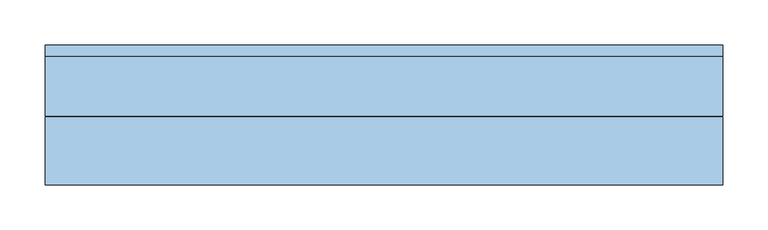
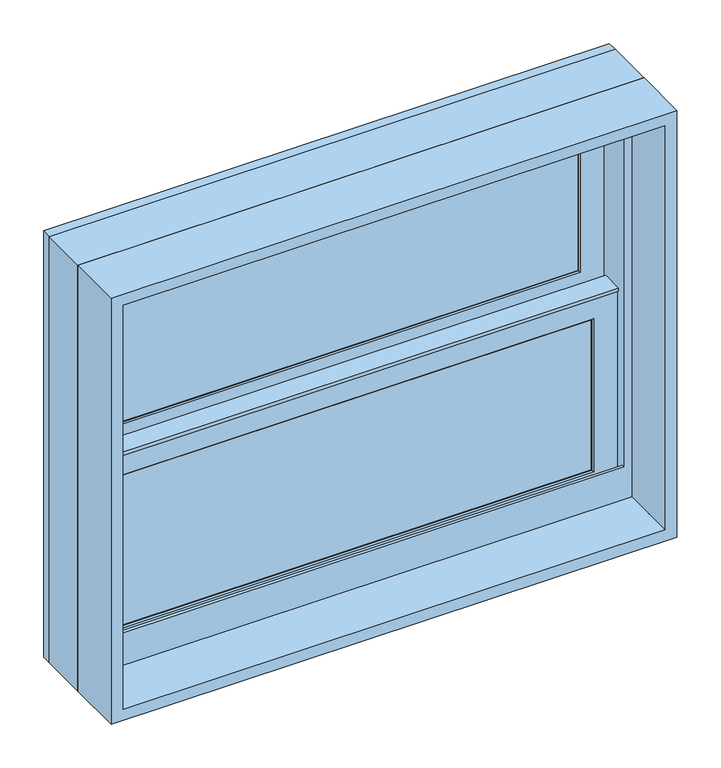
"""IFC4 building model written with IfcOpenShell, lengths in millimetres: window geometry, Window-Double_Hung-Marvin-Essential : ESDH2620."""

from ifc_helpers import new_model, si_unit, frame, origin, place, context, project, spatial, polyline, outline, extrude, faceted_brep, source, transform, mapped, element, save


def window_aca55058(model_context):
    return source(origin(), model_context, "Body", "SolidModel", [
        extrude(outline(polyline([(115.3583333, 20.6375), (115.3583333, 15.875), (96.3083333, 15.875), (96.3083333, 20.6375), (115.3583333, 20.6375)])), frame((0.0, 0.0, 1898.65), z_axis=(0.0, 0.0, 1.0), x_axis=(1.0, 0.0, 0.0)), (0.0, 0.0, 1.0), 222.25),
        extrude(outline(polyline([(-96.3083333, 20.6375), (-96.3083333, 15.875), (-115.3583333, 15.875), (-115.3583333, 20.6375), (-96.3083333, 20.6375)])), frame((0.0, 0.0, 1898.65), z_axis=(0.0, 0.0, 1.0), x_axis=(1.0, 0.0, 0.0)), (0.0, 0.0, 1.0), 222.25),
        extrude(outline(polyline([(317.5, 20.6375), (317.5, 15.875), (-317.5, 15.875), (-317.5, 20.6375), (317.5, 20.6375)])), frame((0.0, 0.0, 2000.25), z_axis=(0.0, 0.0, 1.0), x_axis=(1.0, 0.0, 0.0)), (0.0, 0.0, 1.0), 19.05),
        extrude(outline(polyline([(-115.3583333, 46.83125), (-115.3583333, 51.59375), (-96.3083333, 51.59375), (-96.3083333, 46.83125), (-115.3583333, 46.83125)])), frame((0.0, 0.0, 2159.0), z_axis=(0.0, 0.0, 1.0), x_axis=(1.0, 0.0, 0.0)), (0.0, 0.0, 1.0), 222.25),
        extrude(outline(polyline([(96.3083333, 46.83125), (96.3083333, 51.59375), (115.3583333, 51.59375), (115.3583333, 46.83125), (96.3083333, 46.83125)])), frame((0.0, 0.0, 2159.0), z_axis=(0.0, 0.0, 1.0), x_axis=(1.0, 0.0, 0.0)), (0.0, 0.0, 1.0), 222.25),
        extrude(outline(polyline([(-317.5, 46.83125), (-317.5, 51.59375), (317.5, 51.59375), (317.5, 46.83125), (-317.5, 46.83125)])), frame((0.0, 0.0, 2260.6), z_axis=(0.0, 0.0, 1.0), x_axis=(1.0, 0.0, 0.0)), (0.0, 0.0, 1.0), 19.05),
        extrude(outline(polyline([(115.3583333, 20.6375), (96.3083333, 20.6375), (96.3083333, 25.4), (115.3583333, 25.4), (115.3583333, 20.6375)])), frame((0.0, 0.0, 1898.65), z_axis=(0.0, 0.0, 1.0), x_axis=(1.0, 0.0, 0.0)), (0.0, 0.0, 1.0), 222.25),
        extrude(outline(polyline([(-96.3083333, 20.6375), (-115.3583333, 20.6375), (-115.3583333, 25.4), (-96.3083333, 25.4), (-96.3083333, 20.6375)])), frame((0.0, 0.0, 1898.65), z_axis=(0.0, 0.0, 1.0), x_axis=(1.0, 0.0, 0.0)), (0.0, 0.0, 1.0), 222.25),
        extrude(outline(polyline([(317.5, 20.6375), (-317.5, 20.6375), (-317.5, 25.4), (317.5, 25.4), (317.5, 20.6375)])), frame((0.0, 0.0, 2000.25), z_axis=(0.0, 0.0, 1.0), x_axis=(1.0, 0.0, 0.0)), (0.0, 0.0, 1.0), 19.05),
        extrude(outline(polyline([(-115.3583333, 56.35625), (-96.3083333, 56.35625), (-96.3083333, 51.59375), (-115.3583333, 51.59375), (-115.3583333, 56.35625)])), frame((0.0, 0.0, 2159.0), z_axis=(0.0, 0.0, 1.0), x_axis=(1.0, 0.0, 0.0)), (0.0, 0.0, 1.0), 222.25),
        extrude(outline(polyline([(96.3083333, 56.35625), (115.3583333, 56.35625), (115.3583333, 51.59375), (96.3083333, 51.59375), (96.3083333, 56.35625)])), frame((0.0, 0.0, 2159.0), z_axis=(0.0, 0.0, 1.0), x_axis=(1.0, 0.0, 0.0)), (0.0, 0.0, 1.0), 222.25),
        extrude(outline(polyline([(-317.5, 56.35625), (317.5, 56.35625), (317.5, 51.59375), (-317.5, 51.59375), (-317.5, 56.35625)])), frame((0.0, 0.0, 2260.6), z_axis=(0.0, 0.0, 1.0), x_axis=(1.0, 0.0, 0.0)), (0.0, 0.0, 1.0), 19.05),
        faceted_brep([(-344.4875, 5.6780605, 2150.9351748), (-344.4875, 5.6780605, 2146.3), (344.4875, 5.6780605, 2146.3), (344.4875, 5.6780605, 2150.9351748), (-344.4875, 34.8118605, 2150.9351748), (344.4875, 34.8118605, 2150.9351748), (344.4875, 34.8118605, 2146.3), (-344.4875, 34.8118605, 2146.3), (-344.4875, 30.1625, 2146.3), (-344.4875, 30.1625, 1871.6625), (-344.4875, 8.9241104, 1871.6625), (-344.4875, 8.9241104, 2146.3), (344.4875, 8.9241104, 2146.3), (344.4875, 30.1625, 2146.3), (344.4875, 8.9241104, 1871.6625), (344.4875, 30.1625, 1871.6625), (-328.6034752, 11.90625, 2132.0034752), (-328.6034752, 30.1625, 2132.0034752), (328.6034752, 30.1625, 2132.0034752), (328.6034752, 11.90625, 2132.0034752), (-311.94375, 10.4662439, 2115.34375), (-311.94375, 11.90625, 2115.34375), (311.94375, 11.90625, 2115.34375), (311.94375, 10.4662439, 2115.34375), (313.4858834, 8.9241104, 2116.8858834), (-313.4858834, 8.9241104, 2116.8858834), (328.6034752, 30.1625, 1887.5465248), (328.6034752, 11.90625, 1887.5465248), (311.94375, 11.90625, 1904.20625), (311.94375, 10.4662439, 1904.20625), (313.4858834, 8.9241104, 1902.6641166), (-328.6034752, 30.1625, 1887.5465248), (-328.6034752, 11.90625, 1887.5465248), (-311.94375, 11.90625, 1904.20625), (-311.94375, 10.4662439, 1904.20625), (-313.4858834, 8.9241104, 1902.6641166)], [[[0, 1, 2, 3]], [[4, 5, 6, 7]], [[1, 0, 4, 7, 8, 9, 10, 11]], [[2, 1, 11, 12]], [[7, 6, 13, 8]], [[3, 2, 12, 14, 15, 13, 6, 5]], [[0, 3, 5, 4]], [[16, 17, 18, 19]], [[20, 21, 22, 23]], [[20, 23, 24, 25]], [[19, 18, 26, 27]], [[23, 22, 28, 29]], [[24, 23, 29, 30]], [[27, 26, 31, 32]], [[29, 28, 33, 34]], [[30, 29, 34, 35]], [[15, 14, 10, 9]], [[15, 9, 8, 13], [18, 17, 31, 26]], [[17, 16, 32, 31]], [[16, 19, 27, 32], [22, 21, 33, 28]], [[21, 20, 34, 33]], [[20, 25, 35, 34]], [[10, 14, 12, 11], [25, 24, 30, 35]]]),
        extrude(outline(polyline([(38.5955581, 2132.0125), (33.5778968, 2132.0125), (33.5778968, 2133.6), (39.9405976, 2133.6), (39.9405976, 2132.0125), (61.515625, 2132.0125), (47.6307501, 2128.6975159), (38.5955581, 2128.6975159), (38.5955581, 2132.0125)])), frame((-344.4875, 0.0, 0.0), z_axis=(1.0, 0.0, 0.0), x_axis=(0.0, 1.0, 0.0)), (0.0, 0.0, 1.0), 688.975),
        faceted_brep([(374.65, 0.0, 1841.5), (374.65, 0.0, 2438.4), (-374.65, 0.0, 2438.4), (-374.65, 0.0, 1841.5), (348.45625, 0.0, 1902.61875), (-348.45625, 0.0, 1902.61875), (-348.45625, 0.0, 2412.20625), (348.45625, 0.0, 2412.20625), (348.45625, 3.96875, 1841.5), (-348.45625, 3.96875, 1841.5), (-348.45625, 3.96875, 1902.61875), (348.45625, 3.96875, 1902.61875), (-374.65, 65.6828125, 1841.5), (-348.45625, 65.6828125, 1841.5), (348.45625, 65.6828125, 1841.5), (374.65, 65.6828125, 1841.5), (-374.65, 65.6828125, 2438.4), (374.65, 65.6828125, 2438.4), (348.45625, 65.6828125, 2412.20625), (-348.45625, 65.6828125, 2412.20625)], [[[0, 1, 2, 3], [4, 5, 6, 7]], [[8, 9, 10, 11]], [[5, 4, 11, 10]], [[0, 3, 12, 13, 9, 8, 14, 15]], [[13, 12, 16, 17, 15, 14, 18, 19]], [[13, 19, 6, 5, 10, 9]], [[7, 6, 19, 18]], [[18, 14, 8, 11, 4, 7]], [[1, 0, 15, 17]], [[2, 1, 17, 16]], [[3, 2, 16, 12]]]),
        faceted_brep([(348.45625, 30.1625, 2139.95), (346.86875, 30.1625, 2139.95), (346.86875, 30.1625, 1865.8544613), (348.45625, 30.1625, 1865.8544613), (-346.86875, 30.1625, 2139.95), (-348.45625, 30.1625, 2139.95), (-348.45625, 30.1625, 1865.8544613), (-346.86875, 30.1625, 1865.8544613), (346.86875, 63.5, 2139.95), (348.45625, 63.5, 2139.95), (348.45625, 63.5, 1859.3743077), (346.86875, 63.5, 1859.3743077), (-348.45625, 63.5, 2139.95), (-346.86875, 63.5, 2139.95), (-346.86875, 63.5, 1859.3743077), (-348.45625, 63.5, 1859.3743077), (359.7108932, 3.96875, 1870.9460105), (359.7108932, 3.96875, 1841.5), (359.7108932, 65.6828125, 1841.5), (359.7108932, 65.6828125, 1858.950012), (-359.7108932, 3.96875, 1841.5), (-359.7108932, 3.96875, 1870.9460105), (-359.7108932, 65.6828125, 1858.950012), (-359.7108932, 65.6828125, 1841.5), (359.7108932, 78.58125, 1856.4428097), (-359.7108932, 78.58125, 1856.4428097), (-357.6971252, 68.2348864, 1858.4539391), (-339.73135, 68.2348864, 1858.4539391), (-339.73135, 65.6828125, 1858.950012), (339.73135, 65.6828125, 1858.950012), (339.73135, 68.2348864, 1858.4539391), (357.6971252, 68.2348864, 1858.4539391), (-374.65, 65.6828125, 1841.5), (-374.65, 78.5948249, 1841.5), (374.65, 78.5948249, 1841.5), (374.65, 65.6828125, 1841.5), (-374.65, 78.58125, 2438.4), (374.65, 78.58125, 2438.4), (359.7108932, 78.58125, 2423.4608932), (-359.7108932, 78.58125, 2423.4608932), (-374.65, 65.6828125, 2438.4), (-357.6971252, 68.2348864, 2421.4471252), (357.6971252, 68.2348864, 2421.4471252), (339.73135, 68.2348864, 2403.48135), (-339.73135, 68.2348864, 2403.48135), (-339.73135, 65.6828125, 2403.48135), (339.73135, 65.6828125, 2403.48135), (374.65, 65.6828125, 2438.4)], [[[0, 1, 2, 3]], [[4, 5, 6, 7]], [[8, 9, 10, 11]], [[12, 13, 14, 15]], [[1, 8, 11, 2]], [[9, 0, 3, 10]], [[1, 0, 9, 8]], [[5, 4, 13, 12]], [[5, 12, 15, 6]], [[13, 4, 7, 14]], [[16, 17, 18, 19]], [[20, 21, 22, 23]], [[24, 25, 26, 27, 28, 22, 21, 16, 19, 29, 30, 31], [3, 2, 11, 10], [7, 6, 15, 14]], [[17, 16, 21, 20]], [[17, 20, 23, 32, 33, 34, 35, 18]], [[34, 33, 36, 37], [25, 24, 38, 39]], [[33, 32, 40, 36]], [[39, 41, 26, 25]], [[41, 42, 31, 30, 43, 44, 27, 26]], [[44, 45, 28, 27]], [[40, 32, 23, 22, 28, 45, 46, 29, 19, 18, 35, 47]], [[36, 40, 47, 37]], [[39, 38, 42, 41]], [[44, 43, 46, 45]], [[34, 37, 47, 35]], [[42, 38, 24, 31]], [[46, 43, 30, 29]]]),
        extrude(outline(polyline([(324.64375, 11.90625), (-324.64375, 11.90625), (-324.64375, 15.08125), (324.64375, 15.08125), (324.64375, 11.90625)])), frame((0.0, 0.0, 1891.50625), z_axis=(0.0, 0.0, 1.0), x_axis=(1.0, 0.0, 0.0)), (0.0, 0.0, 1.0), 236.5375),
        extrude(outline(polyline([(324.64375, 42.8625), (-324.64375, 42.8625), (-324.64375, 46.0375), (324.64375, 46.0375), (324.64375, 42.8625)])), frame((0.0, 0.0, 2151.85625), z_axis=(0.0, 0.0, 1.0), x_axis=(1.0, 0.0, 0.0)), (0.0, 0.0, 1.0), 236.5375),
        faceted_brep([(-311.94375, 31.194477, 2115.34375), (-313.4858834, 32.7366104, 2116.8858834), (313.4858834, 32.7366104, 2116.8858834), (311.94375, 31.194477, 2115.34375), (-311.94375, 30.1625, 2115.34375), (311.94375, 30.1625, 2115.34375), (-344.4875, 32.7366104, 2147.8875), (-344.4875, 30.1625, 2147.8875), (344.4875, 30.1625, 2147.8875), (344.4875, 32.7366104, 2147.8875), (313.4858834, 32.7366104, 1902.6641166), (311.94375, 31.194477, 1904.20625), (311.94375, 30.1625, 1904.20625), (344.4875, 30.1625, 1871.6625), (344.4875, 32.7366104, 1871.6625), (-313.4858834, 32.7366104, 1902.6641166), (-311.94375, 31.194477, 1904.20625), (-311.94375, 30.1625, 1904.20625), (-344.4875, 30.1625, 1871.6625), (-344.4875, 32.7366104, 1871.6625)], [[[0, 1, 2, 3]], [[4, 0, 3, 5]], [[6, 7, 8, 9]], [[3, 2, 10, 11]], [[5, 3, 11, 12]], [[9, 8, 13, 14]], [[11, 10, 15, 16]], [[12, 11, 16, 17]], [[14, 13, 18, 19]], [[9, 14, 19, 6], [1, 15, 10, 2]], [[16, 15, 1, 0]], [[17, 16, 0, 4]], [[7, 18, 13, 8], [5, 12, 17, 4]], [[19, 18, 7, 6]]]),
        faceted_brep([(-328.6034752, 42.8625, 2392.3534752), (-328.6034752, 61.11875, 2392.3534752), (328.6034752, 61.11875, 2392.3534752), (328.6034752, 42.8625, 2392.3534752), (-311.94375, 41.4224939, 2375.69375), (-311.94375, 42.8625, 2375.69375), (311.94375, 42.8625, 2375.69375), (311.94375, 41.4224939, 2375.69375), (-313.4858834, 39.8803604, 2377.2358834), (313.4858834, 39.8803604, 2377.2358834), (-344.4875, 61.11875, 2408.2375), (-344.4875, 39.8803604, 2408.2375), (344.4875, 39.8803604, 2408.2375), (344.4875, 61.11875, 2408.2375), (328.6034752, 61.11875, 2147.8965248), (328.6034752, 42.8625, 2147.8965248), (311.94375, 42.8625, 2164.55625), (311.94375, 41.4224939, 2164.55625), (313.4858834, 39.8803604, 2163.0141166), (344.4875, 39.8803604, 2132.0125), (344.4875, 61.11875, 2132.0125), (-328.6034752, 61.11875, 2147.8965248), (-328.6034752, 42.8625, 2147.8965248), (-311.94375, 42.8625, 2164.55625), (-311.94375, 41.4224939, 2164.55625), (-313.4858834, 39.8803604, 2163.0141166), (-344.4875, 39.8803604, 2132.0125), (-344.4875, 61.11875, 2132.0125)], [[[0, 1, 2, 3]], [[4, 5, 6, 7]], [[8, 4, 7, 9]], [[10, 11, 12, 13]], [[3, 2, 14, 15]], [[7, 6, 16, 17]], [[9, 7, 17, 18]], [[13, 12, 19, 20]], [[15, 14, 21, 22]], [[17, 16, 23, 24]], [[18, 17, 24, 25]], [[20, 19, 26, 27]], [[13, 20, 27, 10], [1, 21, 14, 2]], [[22, 21, 1, 0]], [[3, 15, 22, 0], [5, 23, 16, 6]], [[24, 23, 5, 4]], [[25, 24, 4, 8]], [[11, 26, 19, 12], [9, 18, 25, 8]], [[27, 26, 11, 10]]]),
        faceted_brep([(-344.4875, 61.11875, 2132.0125), (-344.4875, 63.6928604, 2132.0125), (344.4875, 63.6928604, 2132.0125), (344.4875, 61.11875, 2132.0125), (-311.94375, 62.150727, 2164.55625), (-311.94375, 61.11875, 2164.55625), (311.94375, 61.11875, 2164.55625), (311.94375, 62.150727, 2164.55625), (-313.4858834, 63.6928604, 2163.0141166), (313.4858834, 63.6928604, 2163.0141166), (344.4875, 63.6928604, 2408.2375), (344.4875, 61.11875, 2408.2375), (311.94375, 61.11875, 2375.69375), (311.94375, 62.150727, 2375.69375), (313.4858834, 63.6928604, 2377.2358834), (-344.4875, 63.6928604, 2408.2375), (-344.4875, 61.11875, 2408.2375), (-311.94375, 61.11875, 2375.69375), (-311.94375, 62.150727, 2375.69375), (-313.4858834, 63.6928604, 2377.2358834)], [[[0, 1, 2, 3]], [[4, 5, 6, 7]], [[8, 4, 7, 9]], [[3, 2, 10, 11]], [[7, 6, 12, 13]], [[9, 7, 13, 14]], [[11, 10, 15, 16]], [[13, 12, 17, 18]], [[14, 13, 18, 19]], [[16, 15, 1, 0]], [[3, 11, 16, 0], [5, 17, 12, 6]], [[18, 17, 5, 4]], [[19, 18, 4, 8]], [[1, 15, 10, 2], [9, 14, 19, 8]]]),
        extrude(outline(polyline([(324.64375, 26.19375), (-324.64375, 26.19375), (-324.64375, 30.1625), (324.64375, 30.1625), (324.64375, 26.19375)])), frame((0.0, 0.0, 1891.50625), z_axis=(0.0, 0.0, 1.0), x_axis=(1.0, 0.0, 0.0)), (0.0, 0.0, 1.0), 236.5375),
        extrude(outline(polyline([(324.64375, 57.15), (-324.64375, 57.15), (-324.64375, 61.11875), (324.64375, 61.11875), (324.64375, 57.15)])), frame((0.0, 0.0, 2151.85625), z_axis=(0.0, 0.0, 1.0), x_axis=(1.0, 0.0, 0.0)), (0.0, 0.0, 1.0), 236.5375),
        extrude(outline(polyline([(2438.4, 374.65), (2438.4, -374.65), (1841.5, -374.65), (1841.5, 374.65), (2438.4, 374.65)]), holes=[polyline([(2422.525, 358.775), (1857.375, 358.775), (1857.375, -358.775), (2422.525, -358.775), (2422.525, 358.775)])]), frame((0.0, -76.2, 0.0), z_axis=(0.0, 1.0, 0.0), x_axis=(0.0, 0.0, 1.0)), (0.0, 0.0, 1.0), 75.40625),
    ])


if __name__ == "__main__":
    model = new_model("IFC4")
    model_context = context("Model", 3, world=origin())
    ifc_project = project(units=[si_unit("LENGTHUNIT", "METRE", prefix="MILLI")], contexts=[model_context])
    site = spatial("IfcSite", under=ifc_project)
    building = spatial("IfcBuilding", under=site)
    placement = place(None, origin())
    window_shape = window_aca55058(model_context)
    element("IfcWindow", 1, ObjectType="Window-Double_Hung-Marvin-Essential : ESDH2620", at=placement, inside=building, context=model_context, shape_type="MappedRepresentation", body=[
        mapped(window_shape, transform((0.0, 0.0, 0.0), x_axis=(1.0, 0.0, 0.0), y_axis=(0.0, 1.0, 0.0), z_axis=(0.0, 0.0, 1.0))),
    ])
    save(model, "model.ifc")

# Revit data of these elements
# Type "Window-Double_Hung-Marvin-Essential : ESDH2620"
#   Type Mark = "21"
#   Window Type = "Essential Double Hung"
#   Product data url = "https://bimobject.com/marvin-windows-and-doors/product/marvin-dhwau"
#   Product Guid = "c4a96547-874c-4385-91dc-a058adc19d98"
#   Frame = "All Ultrex"
#   Egress Window = "No"
#   URL = "www.marvin.com"
#   Model = "ESDH2620"
#   Manufacturer = "Marvin Windows and Doors"
#   Label Egress = ""
#   Glass Type = "IG Low E II with Argon"
#   Design Pressure = "DP50"
#   Description = "3024 DBHG"
#   Analytic Construction = "<None>"
#   Prairie Corner Width = 0' - 4"
#   Prairie Corner Height = 0' - 4"
#   Egress Width = 2' - 2 9/16"
#   Egress Height = 0' - 7 27/128"
#   Rough Width = 2' - 6"
#   Rough Height = 2' - 0"
#   Nominal Width = 2' - 6"
#   Nominal Height = 2' - 0"
#   Inset to Installation Flange [instance default] = 0' - 1"
#   Height = 1' - 11 1/2"
#   Egress Area = 1.33014 SF
#   Default Head Height = 8' - 0"
#   Width = 2' - 5 1/2"
#   Daylight Area = 2.83577 SF
#   DLO Width = 2' - 0 9/16"
#   DLO Height = 0' - 8 5/16"
#   Muntins Top Sash = yes
#   Lites Wide Top Sash = 3
#   Lites Wide Bottom Sash = 3
#   Lites High Top Sash = 2
#   Lites High Bottom Sash = 2
#   Lite Cut Prairie 9 = no
#   Lite Cut HV Grid = yes
#   Muntins Bottom Sash = yes
#   Label Visibility = no
#   Jamb Extension Visibility = yes
#   Edition number = 1
#   Interior Material = Ultrex-Marvin-Stonewhite
#   Glazing Material = Glass-Marvin-IG Low E II with Argon
#   Cladding Material = Ultrex-Marvin-Pebblegray
#   Wall Closure = (empty or 0)
#   Assembly Code = ""
# Element 1 (IfcWindow, "Window-Double_Hung-Marvin-Essential : ESDH2620")
#   Materials on its faces: "Ultrex-Marvin-Pebblegray", "Ultrex-Marvin-Stonewhite", "Glass-Marvin-IG Low E II with Argon"
# Materials
#   "Ultrex-Marvin-Stonewhite": class "Paint", colour RGB 250 251 245, transparency 0
#   "Glass-Marvin-IG Low E II with Argon": class "Glass", colour RGB 0 128 192, transparency 0.85
#   "Ultrex-Marvin-Pebblegray": class "Paint", colour RGB 189 185 173, transparency 0
